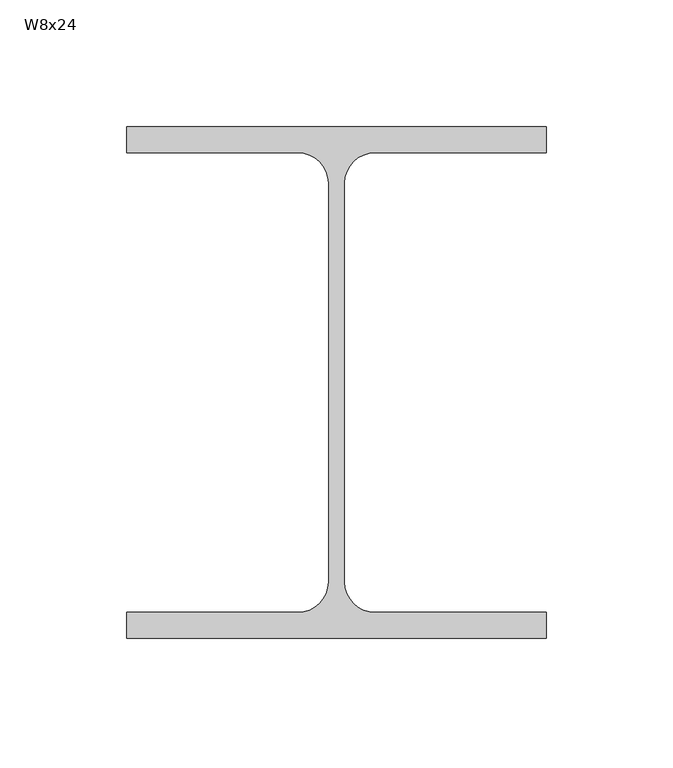
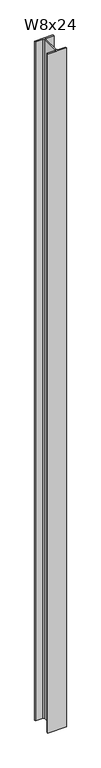
"""IFC4 building model written with IfcOpenShell, lengths in millimetres: column geometry, RME WF - Column : W8x24."""

from ifc_helpers import new_model, si_unit, point, frame, frame_2d, origin, place, context, project, spatial, polyline, circle_curve, trimmed, segment, composite_curve, outline, extrude, source, transform, mapped, element, save


def w8x24_47608c7f(model_context):
    return source(origin(), model_context, "Body", "SweptSolid", [
        extrude(outline(composite_curve([segment(polyline([(82.55, 100.711), (82.55, 90.551), (15.1765, 90.551)]), True, "CONTINUOUS"), segment(trimmed(circle_curve(frame_2d((15.1765, 78.486)), 12.065), [point((15.1765, 90.551))], [point((3.1115, 78.486))], True, "CARTESIAN"), True, "CONTINUOUS"), segment(polyline([(3.1115, 78.486), (3.1115, -78.486)]), True, "CONTINUOUS"), segment(trimmed(circle_curve(frame_2d((15.1765, -78.486)), 12.065), [point((3.1115, -78.486))], [point((15.1765, -90.551))], True, "CARTESIAN"), True, "CONTINUOUS"), segment(polyline([(15.1765, -90.551), (82.55, -90.551), (82.55, -100.711), (-82.55, -100.711), (-82.55, -90.551), (-15.1765, -90.551)]), True, "CONTINUOUS"), segment(trimmed(circle_curve(frame_2d((-15.1765, -78.486)), 12.065), [point((-15.1765, -90.551))], [point((-3.1115, -78.486))], True, "CARTESIAN"), True, "CONTINUOUS"), segment(polyline([(-3.1115, -78.486), (-3.1115, 78.486)]), True, "CONTINUOUS"), segment(trimmed(circle_curve(frame_2d((-15.1765, 78.486)), 12.065), [point((-3.1115, 78.486))], [point((-15.1765, 90.551))], True, "CARTESIAN"), True, "CONTINUOUS"), segment(polyline([(-15.1765, 90.551), (-82.55, 90.551), (-82.55, 100.711), (82.55, 100.711)]), True, "CONTINUOUS")], self_intersect=False)), frame((0.0, 0.0, -304.8), z_axis=(0.0, 0.0, 1.0), x_axis=(1.0, 0.0, 0.0)), (0.0, 0.0, 1.0), 6382.54375),
    ])


if __name__ == "__main__":
    model = new_model("IFC4")
    model_context = context("Model", 3, world=origin())
    ifc_project = project(units=[si_unit("LENGTHUNIT", "METRE", prefix="MILLI")], contexts=[model_context])
    site = spatial("IfcSite", under=ifc_project)
    building = spatial("IfcBuilding", under=site)
    placement = place(None, origin())
    w8x24_shape = w8x24_47608c7f(model_context)
    element("IfcColumn", 1, ObjectType="RME WF - Column : W8x24", at=placement, inside=building, context=model_context, shape_type="MappedRepresentation", body=[
        mapped(w8x24_shape, transform((0.0, 0.0, 0.0), x_axis=(1.0, 0.0, 0.0), y_axis=(0.0, 1.0, 0.0), z_axis=(0.0, 0.0, 1.0))),
    ])
    save(model, "model.ifc")

# Revit data of these elements
# Type "RME WF - Column : W8x24"
#   Type Mark = "C1"
#   REINF TYPE [instance default] = ""
#   Nominal Size = "W16"
#   COL REMARKS [instance default] = ""
#   BP [instance default] = ""
#   Assembly Code = "B10"
#   W = 24
#   bf = 0' - 6 1/2"
#   d = 0' - 7.93"
#   k = 0' - 0 7/8"
#   kr = 0' - 0.475"
#   tf = 0' - 0.4"
#   tw = 0' - 0.245"
#   A = 0.0491667 SF
#   Structural Material [instance default] = Metal - Steel - ASTM A992
# Element 1 (IfcColumn, "RME WF - Column : W8x24")
#   Materials on its faces: "Metal - Steel - ASTM A992"
# Materials
#   "Metal - Steel - ASTM A992": class "Metal", colour RGB 255 128 0, transparency 0
